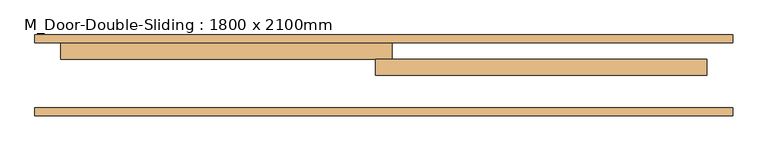
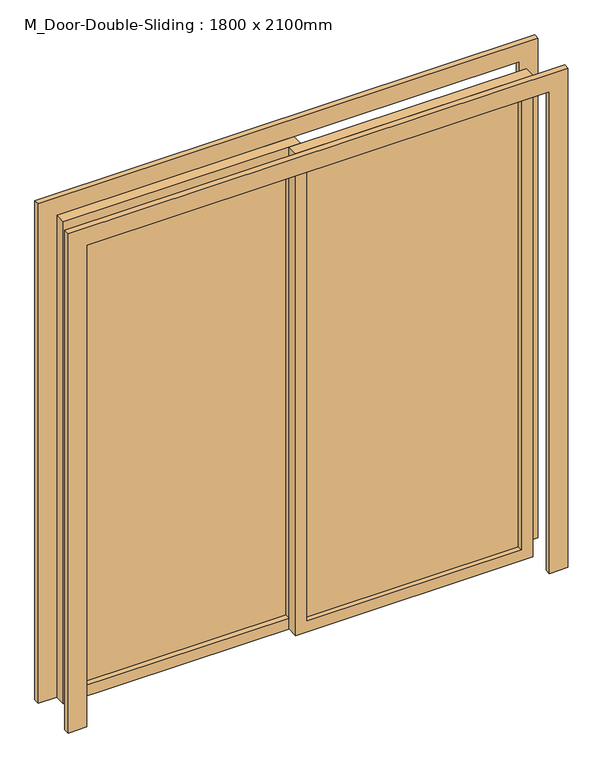
"""IFC4 building model written with IfcOpenShell, lengths in millimetres: door geometry, M_Door-Double-Sliding : 1800 x 2100mm."""

from ifc_helpers import new_model, si_unit, frame, origin, place, context, project, spatial, polyline, outline, extrude, source, transform, mapped, element, save


def m_door_double_sliding_1800_x_2100mm_5b438a36(model_context):
    return source(origin(), model_context, "Body", "SweptSolid", [
        extrude(outline(polyline([(0.0, -1080.0), (0.0, -1000.0), (2200.0, -1000.0), (2200.0, 1000.0), (0.0, 1000.0), (0.0, 1080.0), (2280.0, 1080.0), (2280.0, -1080.0), (0.0, -1080.0)])), frame((0.0, 2.0, 0.0), z_axis=(0.0, 1.0, 0.0), x_axis=(0.0, 0.0, 1.0)), (0.0, 0.0, 1.0), 25.0),
        extrude(outline(polyline([(0.0, 1080.0), (2280.0, 1080.0), (2280.0, -1080.0), (0.0, -1080.0), (0.0, -1000.0), (2200.0, -1000.0), (2200.0, 1000.0), (0.0, 1000.0), (0.0, 1080.0)])), frame((0.0, 227.0, 0.0), z_axis=(0.0, 1.0, 0.0), x_axis=(0.0, 0.0, 1.0)), (0.0, 0.0, 1.0), 25.0),
        extrude(outline(polyline([(2200.0, -25.0), (0.0, -25.0), (0.0, 1000.0), (2200.0, 1000.0), (2200.0, -25.0)]), holes=[polyline([(2150.0, 25.0), (2150.0, 950.0), (50.0, 950.0), (50.0, 25.0), (2150.0, 25.0)])]), frame((0.0, 127.0, 0.0), z_axis=(0.0, 1.0, 0.0), x_axis=(0.0, 0.0, 1.0)), (0.0, 0.0, 1.0), 50.0),
        extrude(outline(polyline([(2200.0, 25.0), (2200.0, -1000.0), (0.0, -1000.0), (0.0, 25.0), (2200.0, 25.0)]), holes=[polyline([(2150.0, -25.0), (50.0, -25.0), (50.0, -950.0), (2150.0, -950.0), (2150.0, -25.0)])]), frame((0.0, 177.0, 0.0), z_axis=(0.0, 1.0, 0.0), x_axis=(0.0, 0.0, 1.0)), (0.0, 0.0, 1.0), 50.0),
        extrude(outline(polyline([(25.0, 155.175), (950.0, 155.175), (950.0, 148.825), (25.0, 148.825), (25.0, 155.175)])), frame((0.0, 0.0, 50.0), z_axis=(0.0, 0.0, 1.0), x_axis=(1.0, 0.0, 0.0)), (0.0, 0.0, 1.0), 2100.0),
        extrude(outline(polyline([(-25.0, 200.025), (-950.0, 200.025), (-950.0, 206.375), (-25.0, 206.375), (-25.0, 200.025)])), frame((0.0, 0.0, 50.0), z_axis=(0.0, 0.0, 1.0), x_axis=(1.0, 0.0, 0.0)), (0.0, 0.0, 1.0), 2100.0),
    ])


if __name__ == "__main__":
    model = new_model("IFC4")
    model_context = context("Model", 3, world=origin())
    ifc_project = project(units=[si_unit("LENGTHUNIT", "METRE", prefix="MILLI")], contexts=[model_context])
    site = spatial("IfcSite", under=ifc_project)
    building = spatial("IfcBuilding", under=site)
    placement = place(None, origin())
    m_door_double_sliding_1800_x_2100mm_shape = m_door_double_sliding_1800_x_2100mm_5b438a36(model_context)
    element("IfcDoor", 1, ObjectType="M_Door-Double-Sliding : 1800 x 2100mm", at=placement, inside=building, context=model_context, shape_type="MappedRepresentation", body=[
        mapped(m_door_double_sliding_1800_x_2100mm_shape, transform((0.0, 0.0, 0.0), x_axis=(1.0, 0.0, 0.0), y_axis=(0.0, 1.0, 0.0), z_axis=(0.0, 0.0, 1.0))),
    ])
    save(model, "model.ifc")

# Revit data of these elements
# Type "M_Door-Double-Sliding : 1800 x 2100mm"
#   Type Mark = "23"
#   Construction Type Id = "opn-d45"
#   Assembly Code = "C1020"
#   Analytic Construction = "Wood frame, double glass door "
#   Thickness = 0.05 m
#   Thermal Resistance (R) = 0.31964 (m²·K)/W
#   Heat Transfer Coefficient (U) = 3.12872 W/(m²·K)
#   Height = 2.2 m
#   Rail Width = 0.05 m
#   Stiles = 0.05 m
#   Trim Projection Ext = 0.025 m
#   Trim Projection Int = 0.025 m
#   Trim Width = 0.08 m
#   Width = 2 m
#   Glazing = Glass
#   Panel Material = Wood - Birch - Solid Stained Light Low Gloss
#   Trim Material = Paint - Sienna
#   Visual Light Transmittance = 0
#   Solar Heat Gain Coefficient = 0
#   Function = (empty or 0)
#   Wall Closure = (empty or 0)
# Element 1 (IfcDoor, "M_Door-Double-Sliding : 1800 x 2100mm")
#   Materials on its faces: "Paint - Sienna", "Wood - Birch - Solid Stained Light Low Gloss", "Glass"
# Materials
#   "Glass": class "Glass", colour RGB 218 227 224, transparency 0.85, Description = "Soda Lime Glass", Cost = 0
#   "Wood - Birch - Solid Stained Light Low Gloss": class "Wood", colour RGB 227 170 128, transparency 0, Cost = 0
#   "Paint - Sienna": class "Miscellaneous", colour RGB 118 70 51, transparency 0, Cost = 0
